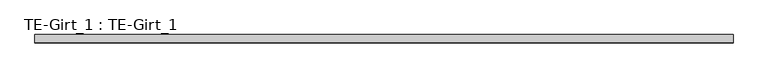
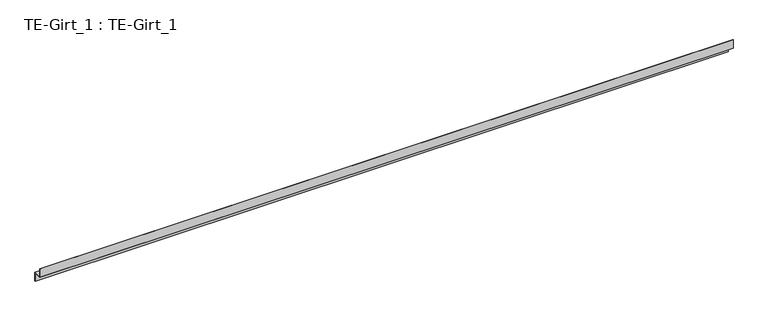
"""IFC4 building model written with IfcOpenShell, lengths in millimetres: proxy geometry, TE-Girt_1 : TE-Girt_1."""

from ifc_helpers import new_model, si_unit, frame, origin, place, context, project, spatial, polyline, outline, extrude, source, transform, mapped, element, save


def te_girt_1_te_girt_1_0389d321(model_context):
    return source(origin(), model_context, "Body", "SweptSolid", [
        extrude(outline(polyline([(-531639.2163841, 844.55), (-531639.2163841, 806.45), (-531640.1093528, 806.45), (-531640.1093528, 843.6570312), (-531674.1249348, 843.6570312), (-531674.1249348, 881.7570312), (-531673.231966, 881.7570312), (-531673.231966, 844.55), (-531639.2163841, 844.55)])), frame((587397.6434739, 0.0, 0.0), z_axis=(1.0, 0.0, 0.0), x_axis=(0.0, 1.0, 0.0)), (0.0, 0.0, 1.0), 2921.0),
    ])


if __name__ == "__main__":
    model = new_model("IFC4")
    model_context = context("Model", 3, world=origin())
    ifc_project = project(units=[si_unit("LENGTHUNIT", "METRE", prefix="MILLI")], contexts=[model_context])
    site = spatial("IfcSite", under=ifc_project)
    building = spatial("IfcBuilding", under=site)
    placement = place(None, origin())
    te_girt_1_te_girt_1_shape = te_girt_1_te_girt_1_0389d321(model_context)
    element("IfcBuildingElementProxy", 1, Name="TE-Girt_1 : TE-Girt_1", ObjectType="TE-Girt_1 : TE-Girt_1", at=placement, inside=building, context=model_context, shape_type="MappedRepresentation", body=[
        mapped(te_girt_1_te_girt_1_shape, transform((0.0, 0.0, 0.0), x_axis=(1.0, 0.0, 0.0), y_axis=(0.0, 1.0, 0.0), z_axis=(0.0, 0.0, 1.0))),
    ])
    save(model, "model.ifc")

# Revit data of these elements
# Element 1 (IfcBuildingElementProxy, "TE-Girt_1 : TE-Girt_1")
#   Materials on its faces: "Z-FURRING, COLD-FORMED GALV."
# Materials
#   "Z-FURRING, COLD-FORMED GALV.": class "Generic", colour RGB 143 142 141, transparency 0, Cost = 0
